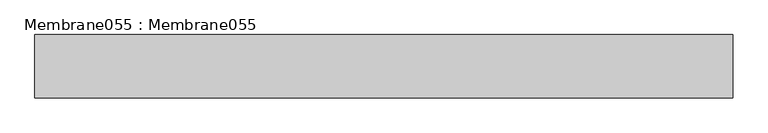
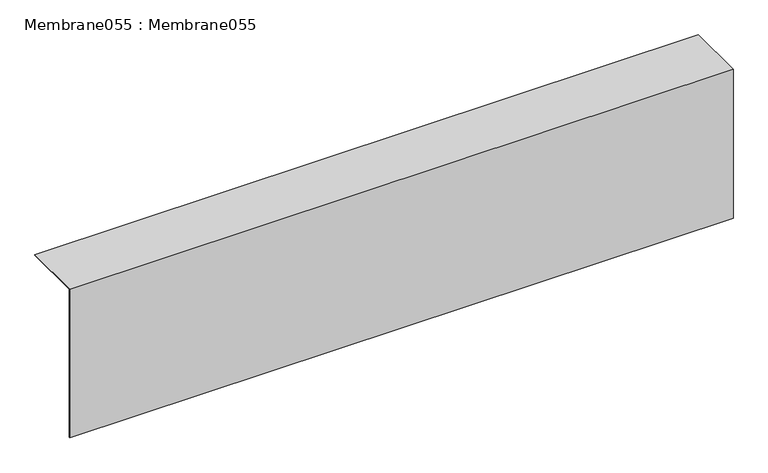
"""IFC4 building model written with IfcOpenShell, lengths in millimetres: proxy geometry, Membrane055 : Membrane055."""

from ifc_helpers import new_model, si_unit, frame, origin, place, context, project, spatial, polyline, outline, extrude, source, transform, mapped, element, save


def membrane055_membrane055_c072a225(model_context):
    return source(origin(), model_context, "Body", "SweptSolid", [
        extrude(outline(polyline([(-5538.3481445, 40223.0071475), (-5538.3481445, 39751.1875), (-5540.3481445, 39751.1875), (-5540.3481445, 40225.0071475), (-5358.6630859, 40225.0071475), (-5358.6630859, 40223.0071475), (-5538.3481445, 40223.0071475)])), frame((12383.0178845, 0.0, 0.0), z_axis=(1.0, 0.0, 0.0), x_axis=(0.0, 1.0, 0.0)), (0.0, 0.0, 1.0), 2000.0),
    ])


if __name__ == "__main__":
    model = new_model("IFC4")
    model_context = context("Model", 3, world=origin())
    ifc_project = project(units=[si_unit("LENGTHUNIT", "METRE", prefix="MILLI")], contexts=[model_context])
    site = spatial("IfcSite", under=ifc_project)
    building = spatial("IfcBuilding", under=site)
    placement = place(None, origin())
    membrane055_membrane055_shape = membrane055_membrane055_c072a225(model_context)
    element("IfcBuildingElementProxy", 1, Name="Membrane055 : Membrane055", ObjectType="Membrane055 : Membrane055", at=placement, inside=building, context=model_context, shape_type="MappedRepresentation", body=[
        mapped(membrane055_membrane055_shape, transform((0.0, 0.0, 0.0), x_axis=(1.0, 0.0, 0.0), y_axis=(0.0, 1.0, 0.0), z_axis=(0.0, 0.0, 1.0))),
    ])
    save(model, "model.ifc")

# Revit data of these elements
# Type "Membrane055 : Membrane055"
#   NameOverride = "Membrane055"
# Element 1 (IfcBuildingElementProxy, "Membrane055 : Membrane055")
#   Materials on its faces: "2 LAYERS NO. 30 ASTM D226 ASPHALT SATURATED ORGANIC FELT"
# Materials
#   "2 LAYERS NO. 30 ASTM D226 ASPHALT SATURATED ORGANIC FELT": class "Unassigned", colour RGB 46 171 0, transparency 0
